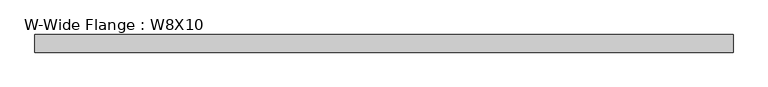
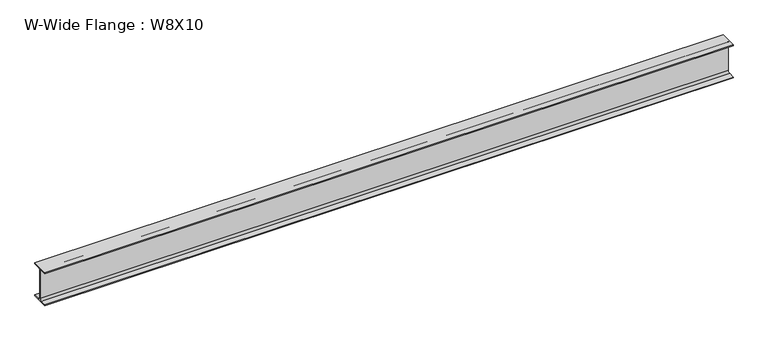
"""IFC4 building model written with IfcOpenShell, lengths in millimetres: beam geometry, W-Wide Flange : W8X10."""

from ifc_helpers import new_model, si_unit, point, frame, frame_2d, origin, place, context, project, spatial, polyline, circle_curve, trimmed, segment, composite_curve, outline, extrude, source, transform, mapped, element, save


def w_wide_flange_w8x10_f96a4068(model_context):
    return source(origin(), model_context, "Body", "SweptSolid", [
        extrude(outline(composite_curve([segment(polyline([(50.038, -94.996), (50.038, -100.203), (-50.038, -100.203), (-50.038, -94.996), (-14.4145, -94.996)]), True, "CONTINUOUS"), segment(trimmed(circle_curve(frame_2d((-14.4145, -82.7405)), 12.2555), [point((-14.4145, -94.996))], [point((-2.159, -82.7405))], True, "CARTESIAN"), True, "CONTINUOUS"), segment(polyline([(-2.159, -82.7405), (-2.159, 82.7405)]), True, "CONTINUOUS"), segment(trimmed(circle_curve(frame_2d((-14.4145, 82.7405)), 12.2555), [point((-2.159, 82.7405))], [point((-14.4145, 94.996))], True, "CARTESIAN"), True, "CONTINUOUS"), segment(polyline([(-14.4145, 94.996), (-50.038, 94.996), (-50.038, 100.203), (50.038, 100.203), (50.038, 94.996), (14.4145, 94.996)]), True, "CONTINUOUS"), segment(trimmed(circle_curve(frame_2d((14.4145, 82.7405)), 12.2555), [point((14.4145, 94.996))], [point((2.159, 82.7405))], True, "CARTESIAN"), True, "CONTINUOUS"), segment(polyline([(2.159, 82.7405), (2.159, -82.7405)]), True, "CONTINUOUS"), segment(trimmed(circle_curve(frame_2d((14.4145, -82.7405)), 12.2555), [point((2.159, -82.7405))], [point((14.4145, -94.996))], True, "CARTESIAN"), True, "CONTINUOUS"), segment(polyline([(14.4145, -94.996), (50.038, -94.996)]), True, "CONTINUOUS")], self_intersect=False)), frame((-1992.5605469, 0.0, 0.0), z_axis=(1.0, 0.0, 0.0), x_axis=(0.0, 1.0, 0.0)), (0.0, 0.0, 1.0), 3956.0440469),
    ])


if __name__ == "__main__":
    model = new_model("IFC4")
    model_context = context("Model", 3, world=origin())
    ifc_project = project(units=[si_unit("LENGTHUNIT", "METRE", prefix="MILLI")], contexts=[model_context])
    site = spatial("IfcSite", under=ifc_project)
    building = spatial("IfcBuilding", under=site)
    placement = place(None, origin())
    w_wide_flange_w8x10_shape = w_wide_flange_w8x10_f96a4068(model_context)
    element("IfcBeam", 1, ObjectType="W-Wide Flange : W8X10", at=placement, inside=building, context=model_context, shape_type="MappedRepresentation", body=[
        mapped(w_wide_flange_w8x10_shape, transform((0.0, 0.0, 0.0), x_axis=(1.0, 0.0, 0.0), y_axis=(0.0, 1.0, 0.0), z_axis=(0.0, 0.0, 1.0))),
    ])
    save(model, "model.ifc")

# Revit data of these elements
# Type "W-Wide Flange : W8X10"
#   Assembly Code = "B10"
#   W = 10
#   Length [instance default] = 1524 mm
#   bf = 100.076 mm
#   d = 200.406 mm
#   k = 17.463 mm
#   k2 = 12.255 mm
#   tf = 5.207 mm
#   tw = 4.318 mm
#   A = 0.00190967 m²
#   Structural Material [instance default] = Steel ASTM A992
# Element 1 (IfcBeam, "W-Wide Flange : W8X10")
#   Structural Material = Aluminum, Anodized Red
#   Materials on its faces: "Aluminum, Anodized Red"
# Materials
#   "Steel ASTM A992": class "Metal", colour RGB 128 0 0, transparency 0, Description = "Structural steel 50ksi", Cost = 0
#   "Aluminum, Anodized Red": class "Metal", colour RGB 120 120 120, transparency 0, Description = "Anodized aluminum, red", Cost = 0
